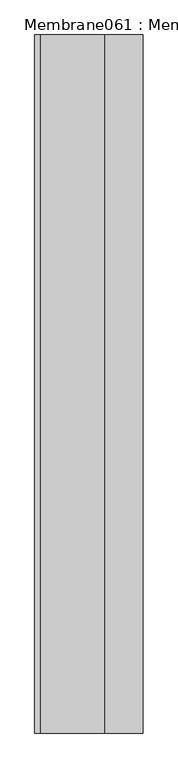
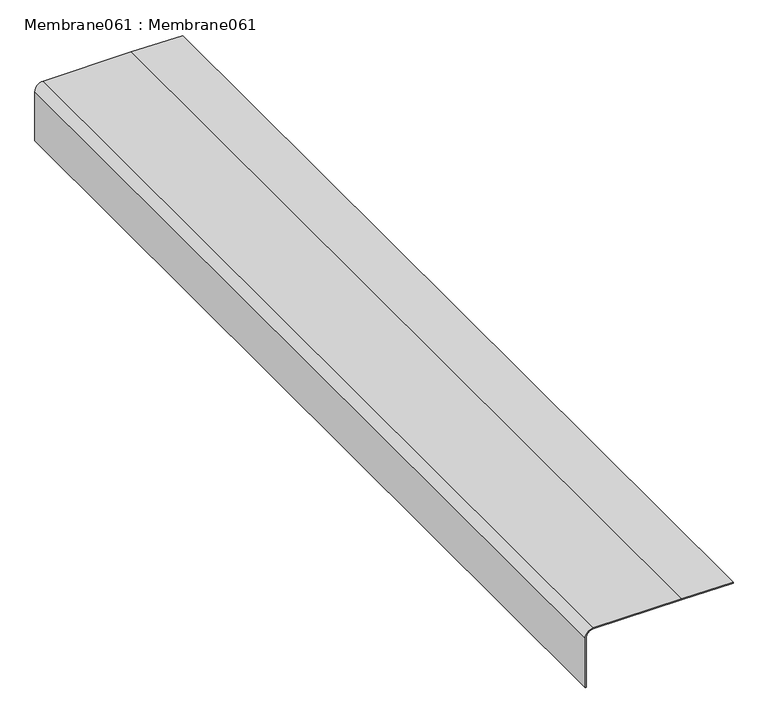
"""IFC4 building model written with IfcOpenShell, lengths in millimetres: proxy geometry, Membrane061 : Membrane061."""

from ifc_helpers import new_model, si_unit, point, frame, frame_2d, origin, place, context, project, spatial, polyline, circle_curve, trimmed, segment, composite_curve, outline, extrude, source, transform, mapped, element, save


def membrane061_membrane061_dffb5b7f(model_context):
    return source(origin(), model_context, "Body", "SweptSolid", [
        extrude(outline(composite_curve([segment(trimmed(circle_curve(frame_2d((40234.8417335, -4992.8194499)), 15.0), [point((40234.8417335, -5007.8194499))], [point((40249.8417335, -4992.8194499))], True, "CARTESIAN"), True, "CONTINUOUS"), segment(polyline([(40249.8417335, -4992.8194499), (40249.8417335, -4807.9081377), (40248.2859925, -4699.8063764), (40250.2861996, -4699.8063764), (40251.8417335, -4807.893747), (40251.8417335, -4992.8194499)]), True, "CONTINUOUS"), segment(trimmed(circle_curve(frame_2d((40234.8417335, -4992.8194499)), 17.0), [point((40251.8417335, -4992.8194499))], [point((40234.8417335, -5009.8194499))], False, "CARTESIAN"), True, "CONTINUOUS"), segment(polyline([(40234.8417335, -5009.8194499), (40125.2457074, -5009.8194499), (40125.2457074, -5007.8194499), (40234.8417335, -5007.8194499)]), True, "CONTINUOUS")], self_intersect=False)), frame((0.0, -1052.8906574, 0.0), z_axis=(0.0, 1.0, 0.0), x_axis=(0.0, 0.0, 1.0)), (0.0, 0.0, 1.0), 2000.0),
    ])


if __name__ == "__main__":
    model = new_model("IFC4")
    model_context = context("Model", 3, world=origin())
    ifc_project = project(units=[si_unit("LENGTHUNIT", "METRE", prefix="MILLI")], contexts=[model_context])
    site = spatial("IfcSite", under=ifc_project)
    building = spatial("IfcBuilding", under=site)
    placement = place(None, origin())
    membrane061_membrane061_shape = membrane061_membrane061_dffb5b7f(model_context)
    element("IfcBuildingElementProxy", 1, Name="Membrane061 : Membrane061", ObjectType="Membrane061 : Membrane061", at=placement, inside=building, context=model_context, shape_type="MappedRepresentation", body=[
        mapped(membrane061_membrane061_shape, transform((0.0, 0.0, 0.0), x_axis=(1.0, 0.0, 0.0), y_axis=(0.0, 1.0, 0.0), z_axis=(0.0, 0.0, 1.0))),
    ])
    save(model, "model.ifc")

# Revit data of these elements
# Type "Membrane061 : Membrane061"
#   NameOverride = "Membrane061"
# Element 1 (IfcBuildingElementProxy, "Membrane061 : Membrane061")
#   Materials on its faces: "THREE PLY BUILT UP ROOF MEMBRANE"
# Materials
#   "THREE PLY BUILT UP ROOF MEMBRANE": class "Unassigned", colour RGB 63 63 63, transparency 0
